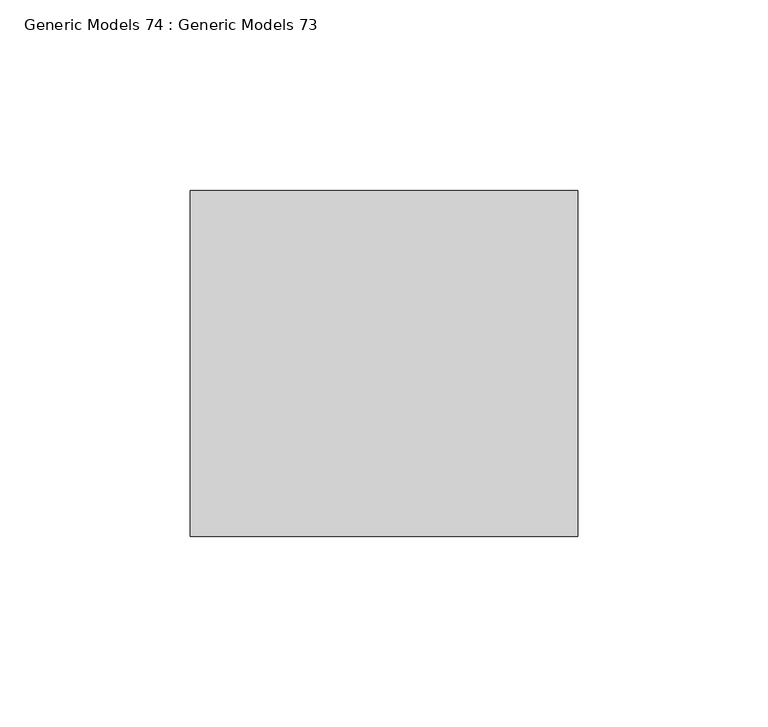
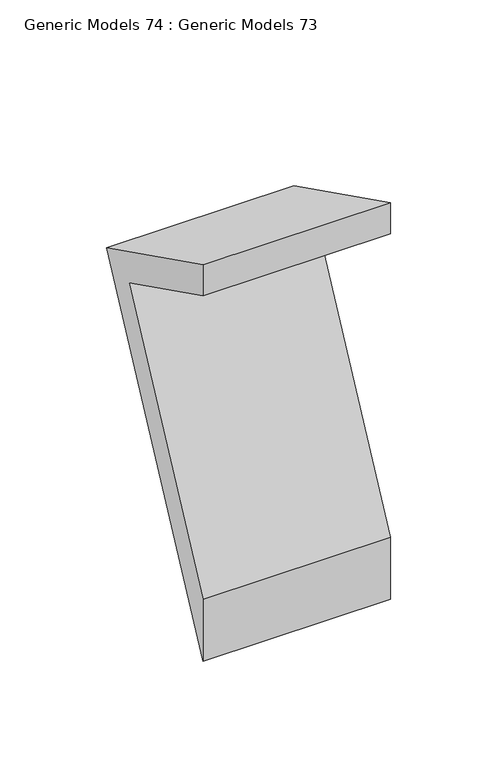
"""IFC4 building model written with IfcOpenShell, lengths in millimetres: proxy geometry, Generic Models 74 : Generic Models 73."""

from ifc_helpers import new_model, si_unit, frame, origin, place, context, project, spatial, polyline, outline, extrude, source, transform, mapped, element, save


def generic_models_74_generic_models_73_a4c67aa6(model_context):
    return source(origin(), model_context, "Body", "SweptSolid", [
        extrude(outline(polyline([(30943.0019638, 271652.1851052), (30852.1281612, 271470.4375), (30852.1281612, 271505.9350791), (30921.7034163, 271645.0855894), (30852.1281612, 271679.8732169), (30852.1281612, 271697.6220065), (30943.0019638, 271652.1851052)])), frame((31924.6096032, 0.0, 0.0), z_axis=(1.0, 0.0, 0.0), x_axis=(0.0, 1.0, 0.0)), (0.0, 0.0, 1.0), 101.6),
    ])


if __name__ == "__main__":
    model = new_model("IFC4")
    model_context = context("Model", 3, world=origin())
    ifc_project = project(units=[si_unit("LENGTHUNIT", "METRE", prefix="MILLI")], contexts=[model_context])
    site = spatial("IfcSite", under=ifc_project)
    building = spatial("IfcBuilding", under=site)
    placement = place(None, origin())
    generic_models_74_generic_models_73_shape = generic_models_74_generic_models_73_a4c67aa6(model_context)
    element("IfcBuildingElementProxy", 1, Name="Generic Models 74 : Generic Models 73", ObjectType="Generic Models 74 : Generic Models 73", at=placement, inside=building, context=model_context, shape_type="MappedRepresentation", body=[
        mapped(generic_models_74_generic_models_73_shape, transform((0.0, 0.0, 0.0), x_axis=(1.0, 0.0, 0.0), y_axis=(0.0, 1.0, 0.0), z_axis=(0.0, 0.0, 1.0))),
    ])
    save(model, "model.ifc")

# Revit data of these elements
# Element 1 (IfcBuildingElementProxy, "Generic Models 74 : Generic Models 73")
#   Materials on its faces: "L8 x 4 x 5/8 x 0'-4\" METAL ANGLE"
# Materials
#   "L8 x 4 x 5/8 x 0'-4\" METAL ANGLE": class "Metal", colour RGB 199 199 199, transparency 0, Description = "Carbon steel", Cost = 0
